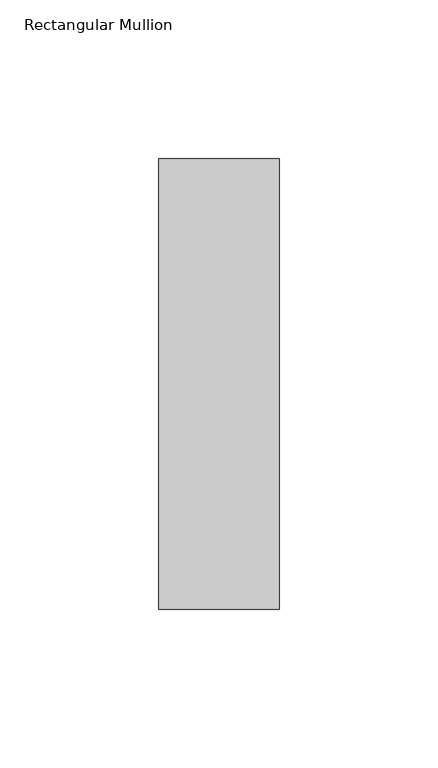
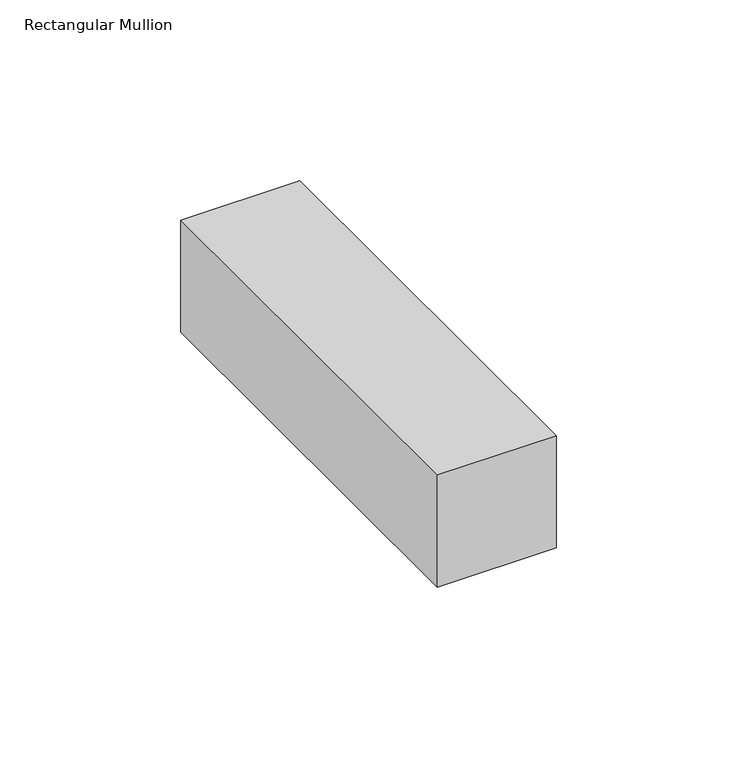
"""IFC4 building model written with IfcOpenShell, lengths in millimetres: member geometry, Rectangular Mullion : NLRS_21_CWM_hsb-regel 38x142_gen_rsf."""

from ifc_helpers import new_model, si_unit, frame, origin, place, context, project, spatial, polyline, outline, extrude, source, transform, mapped, element, save


def rectangular_mullion_ad49c1d0(model_context):
    return source(origin(), model_context, "Body", "SweptSolid", [
        extrude(outline(polyline([(-38.0, -71.0), (-38.0, 71.0), (0.0, 71.0), (0.0, -71.0), (-38.0, -71.0)])), frame((0.0, 0.0, -38.0), z_axis=(0.0, 0.0, 1.0), x_axis=(1.0, 0.0, 0.0)), (0.0, 0.0, 1.0), 38.0),
    ])


if __name__ == "__main__":
    model = new_model("IFC4")
    model_context = context("Model", 3, world=origin())
    ifc_project = project(units=[si_unit("LENGTHUNIT", "METRE", prefix="MILLI")], contexts=[model_context])
    site = spatial("IfcSite", under=ifc_project)
    building = spatial("IfcBuilding", under=site)
    placement = place(None, origin())
    rectangular_mullion_shape = rectangular_mullion_ad49c1d0(model_context)
    element("IfcMember", 1, ObjectType="Rectangular Mullion : NLRS_21_CWM_hsb-regel 38x142_gen_rsf", at=placement, inside=building, context=model_context, shape_type="MappedRepresentation", body=[
        mapped(rectangular_mullion_shape, transform((0.0, 0.0, 0.0), x_axis=(1.0, 0.0, 0.0), y_axis=(0.0, 1.0, 0.0), z_axis=(0.0, 0.0, 1.0))),
    ])
    save(model, "model.ifc")

# Revit data of these elements
# Type "Rectangular Mullion : NLRS_21_CWM_hsb-regel 38x142_gen_rsf"
#   Export Type to IFC As = "IfcWall"
#   Type IfcGUID = "07M7mRoiH1CR8m_RSKIwpF"
#   Assembly Code = "21.10"
#   built-in parameter 1007322 = 0.465879 (stored number, unit not read)
#   built-in parameter 1007321 = 0.062336 (stored number, unit not read)
#   built-in parameter 1007320 = 0.062336 (stored number, unit not read)
# Element 1 (IfcMember, "Rectangular Mullion : NLRS_21_CWM_hsb-regel 38x142_gen_rsf")
#   Materials on its faces: "NLRS_i2_hout naaldhout vuren_gen_rsf"
# Materials
#   "NLRS_i2_hout naaldhout vuren_gen_rsf": class "I - Hout", colour RGB 234 199 147, transparency 0, Keynote = "i2", Manufacturer = "Revit Standards Foundation", URL = "www.revitstandards.org", Description = "hout vuren", Cost = 0
